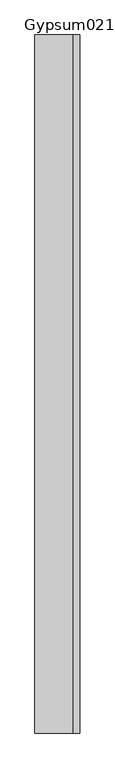
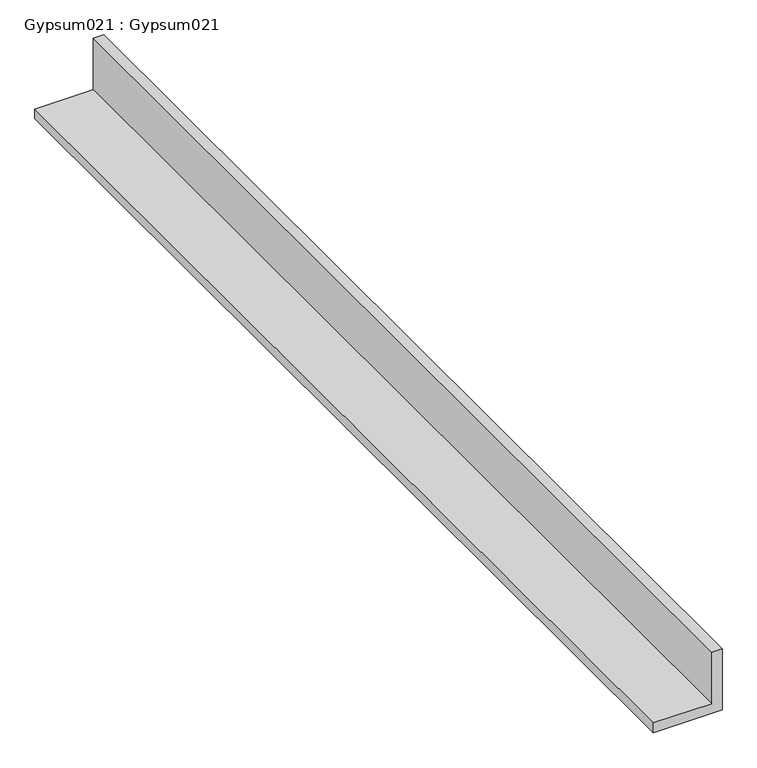
"""IFC4 building model written with IfcOpenShell, lengths in millimetres: proxy geometry, Gypsum021 : Gypsum021."""

from ifc_helpers import new_model, si_unit, frame, origin, place, context, project, spatial, polyline, outline, extrude, source, transform, mapped, element, save


def gypsum021_gypsum021_68a84911(model_context):
    return source(origin(), model_context, "Body", "SweptSolid", [
        extrude(outline(polyline([(42032.2036692, -950.3815411), (42032.2036692, -1059.7768555), (42013.1536692, -1059.7768555), (42013.1536692, -931.3315411), (42133.8036692, -931.3315411), (42133.8036692, -950.3815411), (42032.2036692, -950.3815411)])), frame((0.0, -1052.8906574, 0.0), z_axis=(0.0, 1.0, 0.0), x_axis=(0.0, 0.0, 1.0)), (0.0, 0.0, 1.0), 2000.0),
    ])


if __name__ == "__main__":
    model = new_model("IFC4")
    model_context = context("Model", 3, world=origin())
    ifc_project = project(units=[si_unit("LENGTHUNIT", "METRE", prefix="MILLI")], contexts=[model_context])
    site = spatial("IfcSite", under=ifc_project)
    building = spatial("IfcBuilding", under=site)
    placement = place(None, origin())
    gypsum021_gypsum021_shape = gypsum021_gypsum021_68a84911(model_context)
    element("IfcBuildingElementProxy", 1, Name="Gypsum021 : Gypsum021", ObjectType="Gypsum021 : Gypsum021", at=placement, inside=building, context=model_context, shape_type="MappedRepresentation", body=[
        mapped(gypsum021_gypsum021_shape, transform((0.0, 0.0, 0.0), x_axis=(1.0, 0.0, 0.0), y_axis=(0.0, 1.0, 0.0), z_axis=(0.0, 0.0, 1.0))),
    ])
    save(model, "model.ifc")

# Revit data of these elements
# Type "Gypsum021 : Gypsum021"
#   NameOverride = "Gypsum021"
# Element 1 (IfcBuildingElementProxy, "Gypsum021 : Gypsum021")
#   Materials on its faces: "5/8\" GYPSUM BOARD"
# Materials
#   "5/8\" GYPSUM BOARD": class "Unassigned", colour RGB 255 255 255, transparency 0, Cost = 0
